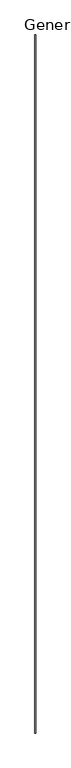
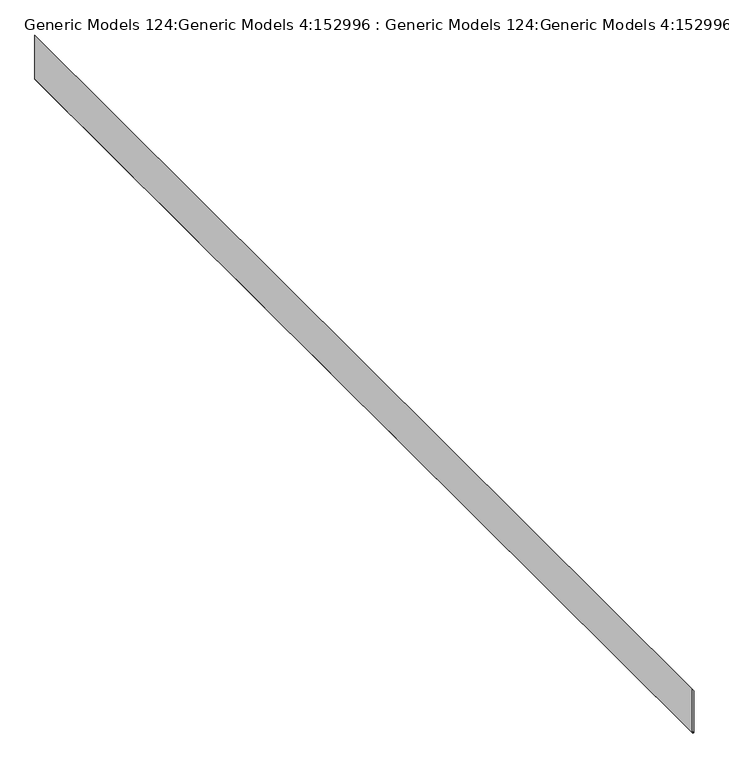
"""IFC4 building model written with IfcOpenShell, lengths in millimetres: proxy geometry, Generic Models 124:Generic Models 4:152996 : Generic Models 124:Generic Models 4:152996."""

from ifc_helpers import new_model, si_unit, frame, origin, place, context, project, spatial, polyline, outline, extrude, source, transform, mapped, element, save


def generic_models_124_generic_models_4_152996_generic_models_d4044557(model_context):
    return source(origin(), model_context, "Body", "SweptSolid", [
        extrude(outline(polyline([(3046.095, 7033.773213), (3046.095, 7051.6443374), (3770.9747574, 7051.6443374), (3808.2495785, 7032.503213), (3049.5748, 7032.503213), (3049.5748, 7033.3620539), (3068.6193787, 7033.3620539), (3068.6193787, 7034.6320539), (3048.3048, 7034.6320539), (3048.3048, 7033.773213), (3046.095, 7033.773213)])), frame((0.0, -6674.7974793, 0.0), z_axis=(0.0, 1.0, 0.0), x_axis=(0.0, 0.0, 1.0)), (0.0, 0.0, 1.0), 18643.6),
    ])


if __name__ == "__main__":
    model = new_model("IFC4")
    model_context = context("Model", 3, world=origin())
    ifc_project = project(units=[si_unit("LENGTHUNIT", "METRE", prefix="MILLI")], contexts=[model_context])
    site = spatial("IfcSite", under=ifc_project)
    building = spatial("IfcBuilding", under=site)
    placement = place(None, origin())
    generic_models_124_generic_models_4_152996_generic_models_shape = generic_models_124_generic_models_4_152996_generic_models_d4044557(model_context)
    element("IfcBuildingElementProxy", 1, Name="Generic Models 124:Generic Models 4:152996 : Generic Models 124:Generic Models 4:152996", ObjectType="Generic Models 124:Generic Models 4:152996 : Generic Models 124:Generic Models 4:152996", at=placement, inside=building, context=model_context, shape_type="MappedRepresentation", body=[
        mapped(generic_models_124_generic_models_4_152996_generic_models_shape, transform((0.0, 0.0, 0.0), x_axis=(1.0, 0.0, 0.0), y_axis=(0.0, 1.0, 0.0), z_axis=(0.0, 0.0, 1.0))),
    ])
    save(model, "model.ifc")

# Revit data of these elements
# Type "Generic Models 124:Generic Models 4:152996 : Generic Models 124:Generic Models 4:152996"
#   NameOverride = "Generic Models 124:Generic Models 4:152996"
#   ObjectTypeOverride = "Generic Models 124:Generic Models 4"
#   Reference = "Generic Models 4"
#   Category = "Generic Models"
#   Tag = "152996"
# Element 1 (IfcBuildingElementProxy, "Generic Models 124:Generic Models 4:152996 : Generic Models 124:Generic Models 4:152996")
#   Materials on its faces: "_7/8\" SMOOTH TROWEL EXTERIOR STUCCO (COLOR PER OWNER) 770"
# Materials
#   "_7/8\" SMOOTH TROWEL EXTERIOR STUCCO (COLOR PER OWNER) 770": class "Unassigned", colour RGB 233 233 233, transparency 0
